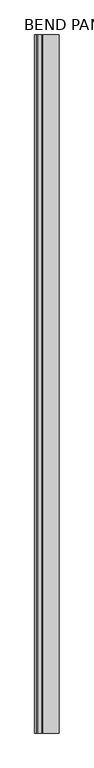
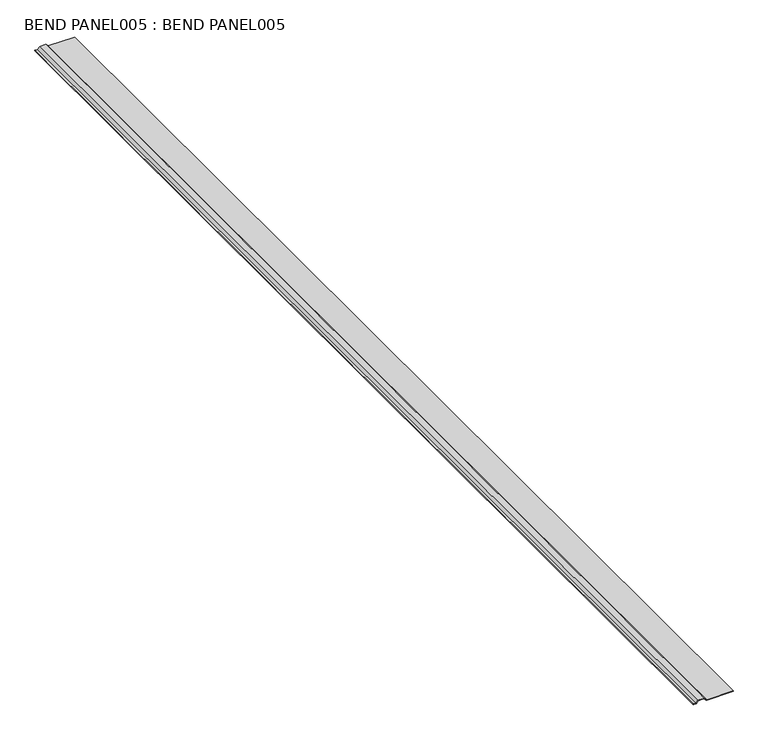
"""IFC4 building model written with IfcOpenShell, lengths in millimetres: proxy geometry, BEND PANEL005 : BEND PANEL005."""

import ifcopenshell
import ifcopenshell.guid

model = None  # the IFC model being written
_history = None  # IfcOwnerHistory: only IFC2X3 demands one
_inside = {}  # id of a spatial element -> (the spatial element, [elements in it])
_under = {}  # id of a project, library or spatial element -> (it, [spatial elements below it])
_declared = {}  # id of a project -> (the project, [libraries it declares])
_typed = {}  # id of a type object -> (the type object, [elements of that type])
_made_of = {}  # id of a material, layer set ... -> (it, [elements and type objects made of it])


def new_model(schema):
    """Start an empty IFC model of exactly this schema.

    Asked for "IFC4X3", IfcOpenShell would pick the latest addendum, in which some entities
    have other attributes; the version numbers below select the first issue.
    IFC2X3 requires an IfcOwnerHistory on every rooted entity: one is made here for all.
    """
    global model, _history
    if schema == "IFC4X3":
        model = ifcopenshell.file(schema_version=(4, 3, 0, 0))
    else:
        model = ifcopenshell.file(schema=schema)
    _inside.clear()
    _under.clear()
    _declared.clear()
    _typed.clear()
    _made_of.clear()
    _history = None
    if model.schema == "IFC2X3":
        org = make("IfcOrganization", Name="unknown")
        user = make(
            "IfcPersonAndOrganization",
            ThePerson=make("IfcPerson", FamilyName="unknown"),
            TheOrganization=org,
        )
        app = make(
            "IfcApplication",
            ApplicationDeveloper=org,
            Version="unknown",
            ApplicationFullName="unknown",
            ApplicationIdentifier="unknown",
        )
        _history = make(
            "IfcOwnerHistory",
            OwningUser=user,
            OwningApplication=app,
            ChangeAction="ADDED",
            CreationDate=0,
        )
    return model


def make(cls, **values):
    """One entity of the class cls with the attributes given. An attribute that is None is left unset."""
    return model.create_entity(
        cls, **{name: value for name, value in values.items() if value is not None}
    )


def rooted(cls, **values):
    """An entity with a GlobalId (a new one), such as an element, a storey or a relation."""
    return make(cls, GlobalId=ifcopenshell.guid.new(), OwnerHistory=_history, **values)


def si_unit(unit_type, name, prefix=None):
    """IfcSIUnit, for example si_unit("LENGTHUNIT", "METRE", prefix="MILLI")."""
    return make("IfcSIUnit", UnitType=unit_type, Prefix=prefix, Name=name)


def assignment(units):
    """IfcUnitAssignment: the units of a project."""
    return None if units is None else make("IfcUnitAssignment", Units=units)


def point(xyz):
    """IfcCartesianPoint."""
    return None if xyz is None else make("IfcCartesianPoint", Coordinates=xyz)


def direction(xyz):
    """IfcDirection."""
    return None if xyz is None else make("IfcDirection", DirectionRatios=xyz)


def frame(location, z_axis=None, x_axis=None):
    """IfcAxis2Placement3D, a coordinate frame: its origin and axes. An axis left out is left unset."""
    return make(
        "IfcAxis2Placement3D",
        Location=point(location),
        Axis=direction(z_axis),
        RefDirection=direction(x_axis),
    )


def frame_2d(location, x_axis=None):
    """IfcAxis2Placement2D, a coordinate frame in the plane: its origin and x axis."""
    return make(
        "IfcAxis2Placement2D", Location=point(location), RefDirection=direction(x_axis)
    )


def origin():
    """The frame at (0, 0, 0) with its axes left unset."""
    return frame((0.0, 0.0, 0.0))


def place(relative_to, where):
    """IfcLocalPlacement: puts the frame where relative to a parent placement (None: the world)."""
    return make(
        "IfcLocalPlacement", PlacementRelTo=relative_to, RelativePlacement=where
    )


def context(
    kind, dimensions, precision=None, world=None, true_north=None, identifier=None
):
    """IfcGeometricRepresentationContext, for example the 3D "Model" context."""
    return make(
        "IfcGeometricRepresentationContext",
        ContextIdentifier=identifier,
        ContextType=kind,
        CoordinateSpaceDimension=dimensions,
        Precision=precision,
        WorldCoordinateSystem=world,
        TrueNorth=true_north,
    )


def project(units=None, contexts=None):
    """IfcProject with its units and contexts."""
    return rooted(
        "IfcProject",
        Name="project",
        RepresentationContexts=contexts,
        UnitsInContext=assignment(units),
    )


def spatial(cls, under=None, at=None, **own):
    """A site, building, storey or space (cls), placed at a placement, below another one or the project."""
    s = rooted(cls, ObjectPlacement=at, **own)
    if under is not None:
        _under.setdefault(under.id(), (under, []))[1].append(s)
    return s


def polyline(points):
    """IfcPolyline through the points."""
    return make("IfcPolyline", Points=[point(p) for p in points])


def circle_curve(where, radius):
    """IfcCircle in the frame where."""
    return make("IfcCircle", Position=where, Radius=radius)


def trimmed(basis, trim1, trim2, sense, master):
    """IfcTrimmedCurve: the piece of a basis curve between two trims."""
    return make(
        "IfcTrimmedCurve",
        BasisCurve=basis,
        Trim1=trim1,
        Trim2=trim2,
        SenseAgreement=sense,
        MasterRepresentation=master,
    )


def segment(curve, same_sense, transition):
    """IfcCompositeCurveSegment."""
    return make(
        "IfcCompositeCurveSegment",
        Transition=transition,
        SameSense=same_sense,
        ParentCurve=curve,
    )


def composite_curve(segments, self_intersect=None):
    """IfcCompositeCurve: segments joined end to end."""
    return make("IfcCompositeCurve", Segments=segments, SelfIntersect=self_intersect)


def outline(outer, holes=None, kind="AREA"):
    """IfcArbitraryClosedProfileDef: a profile drawn as a closed curve; with holes, ...WithVoids."""
    if holes is None:
        return make("IfcArbitraryClosedProfileDef", ProfileType=kind, OuterCurve=outer)
    return make(
        "IfcArbitraryProfileDefWithVoids",
        ProfileType=kind,
        OuterCurve=outer,
        InnerCurves=holes,
    )


def extrude(swept, where, along, depth):
    """IfcExtrudedAreaSolid: the profile swept, set in the frame where, extruded along a direction by depth."""
    return make(
        "IfcExtrudedAreaSolid",
        SweptArea=swept,
        Position=where,
        ExtrudedDirection=direction(along),
        Depth=depth,
    )


def shape(context_of_items, identifier, shape_type, items):
    """IfcShapeRepresentation: the items that make up one representation, for example the "Body"."""
    return make(
        "IfcShapeRepresentation",
        ContextOfItems=context_of_items,
        RepresentationIdentifier=identifier,
        RepresentationType=shape_type,
        Items=items,
    )


def source(mapping_origin, context_of_items, identifier, shape_type, items):
    """IfcRepresentationMap: a shape defined once, which mapped items show again and again."""
    return make(
        "IfcRepresentationMap",
        MappingOrigin=mapping_origin,
        MappedRepresentation=shape(context_of_items, identifier, shape_type, items),
    )


def transform(
    local_origin,
    x_axis=None,
    y_axis=None,
    z_axis=None,
    scale=None,
    scale2=None,
    scale3=None,
    uniform=True,
):
    """IfcCartesianTransformationOperator3D, or its non-uniform kind. x_axis, y_axis, z_axis: its Axis1, 2, 3."""
    if uniform:
        return make(
            "IfcCartesianTransformationOperator3D",
            Axis1=direction(x_axis),
            Axis2=direction(y_axis),
            LocalOrigin=point(local_origin),
            Scale=scale,
            Axis3=direction(z_axis),
        )
    return make(
        "IfcCartesianTransformationOperator3DnonUniform",
        Axis1=direction(x_axis),
        Axis2=direction(y_axis),
        LocalOrigin=point(local_origin),
        Scale=scale,
        Axis3=direction(z_axis),
        Scale2=scale2,
        Scale3=scale3,
    )


def mapped(mapping_source, mapping_target):
    """IfcMappedItem: shows the shape of a source again, moved by a transform."""
    return make(
        "IfcMappedItem", MappingSource=mapping_source, MappingTarget=mapping_target
    )


def made_of(thing, what):
    """Note that an element or type object is made of a material, layer set ...; save() writes the relation."""
    if what is not None:
        _made_of.setdefault(what.id(), (what, []))[1].append(thing)
    return thing


def element(
    cls,
    number,
    at=None,
    inside=None,
    cuts=None,
    type_object=None,
    material=None,
    context=None,
    identifier="Body",
    shape_type=None,
    held_by="IfcProductDefinitionShape",
    body=None,
    shapes=None,
    **own,
):
    """One element of the class cls, such as IfcWall. Its Tag is "e" and its number.

    at: its placement. inside: the storey or other place that contains it. cuts: it is an
    opening in that element (IfcRelVoidsElement). A single representation is given by context,
    identifier, shape_type and body (its items); several are given by shapes. held_by: the class
    of the entity that holds the representations. save() writes the other relations.
    """
    e = rooted(cls, Tag="e%d" % number, ObjectPlacement=at, **own)
    if body is not None:
        shapes = [shape(context, identifier, shape_type, body)]
    if shapes is not None:
        e.Representation = make(held_by, Representations=shapes)
    if inside is not None:
        _inside.setdefault(inside.id(), (inside, []))[1].append(e)
    if cuts is not None:
        rooted(
            "IfcRelVoidsElement", RelatingBuildingElement=cuts, RelatedOpeningElement=e
        )
    if type_object is not None:
        _typed.setdefault(type_object.id(), (type_object, []))[1].append(e)
    return made_of(e, material)


def aggregate(whole, parts):
    """IfcRelAggregates: a whole, such as a stair, and the parts it consists of."""
    return rooted("IfcRelAggregates", RelatingObject=whole, RelatedObjects=parts)


def save(model, path):
    """Write the relations noted so far, then the file.

    IfcRelAggregates (storeys below a building ...), IfcRelContainedInSpatialStructure (elements
    in a storey), IfcRelDefinesByType, IfcRelAssociatesMaterial and IfcRelDeclares: one each for
    every whole, place, type object, material and project.
    """
    for whole, parts in _under.values():
        aggregate(whole, parts)
    for where, things in _inside.values():
        rooted(
            "IfcRelContainedInSpatialStructure",
            RelatedElements=things,
            RelatingStructure=where,
        )
    for kind, things in _typed.values():
        rooted("IfcRelDefinesByType", RelatedObjects=things, RelatingType=kind)
    for what, things in _made_of.values():
        rooted("IfcRelAssociatesMaterial", RelatedObjects=things, RelatingMaterial=what)
    for by, libraries in _declared.values():
        rooted("IfcRelDeclares", RelatingContext=by, RelatedDefinitions=libraries)
    model.write(path)


def bend_panel005_bend_panel005_8c87a596(model_context):
    return source(origin(), model_context, "Body", "SweptSolid", [
        extrude(outline(composite_curve([segment(polyline([(42575.4212949, 5895.2230694), (42576.6119199, 5895.2230694), (42576.6119199, 5848.7155886), (42580.7948046, 5844.5327039), (42580.7948046, 5833.5642507), (42576.6119199, 5829.381366), (42576.6119199, 5825.5083246), (42575.4212949, 5825.5083246), (42575.4212949, 5829.381366)]), True, "CONTINUOUS"), segment(trimmed(circle_curve(frame_2d((42576.6119199, 5829.381366)), 1.190625), [point((42575.4212949, 5829.381366))], [point((42575.7700209, 5830.223265))], False, "CARTESIAN"), True, "CONTINUOUS"), segment(polyline([(42575.7700209, 5830.223265), (42579.6041796, 5834.0574237), (42579.6041796, 5844.0395308), (42575.7700209, 5847.8736895)]), True, "CONTINUOUS"), segment(trimmed(circle_curve(frame_2d((42576.6119199, 5848.7155885)), 1.190625), [point((42575.7700209, 5847.8736895))], [point((42575.4212949, 5848.7155885))], False, "CARTESIAN"), True, "CONTINUOUS"), segment(polyline([(42575.4212949, 5848.7155885), (42575.4212949, 5895.2230694)]), True, "CONTINUOUS")], self_intersect=False)), frame((0.0, -1052.8906574, 0.0), z_axis=(0.0, 1.0, 0.0), x_axis=(0.0, 0.0, 1.0)), (0.0, 0.0, 1.0), 1999.85),
    ])


if __name__ == "__main__":
    model = new_model("IFC4")
    model_context = context("Model", 3, world=origin())
    ifc_project = project(units=[si_unit("LENGTHUNIT", "METRE", prefix="MILLI")], contexts=[model_context])
    site = spatial("IfcSite", under=ifc_project)
    building = spatial("IfcBuilding", under=site)
    placement = place(None, origin())
    bend_panel005_bend_panel005_shape = bend_panel005_bend_panel005_8c87a596(model_context)
    element("IfcBuildingElementProxy", 1, Name="BEND PANEL005 : BEND PANEL005", ObjectType="BEND PANEL005 : BEND PANEL005", at=placement, inside=building, context=model_context, shape_type="MappedRepresentation", body=[
        mapped(bend_panel005_bend_panel005_shape, transform((0.0, 0.0, 0.0), x_axis=(1.0, 0.0, 0.0), y_axis=(0.0, 1.0, 0.0), z_axis=(0.0, 0.0, 1.0))),
    ])
    save(model, "model.ifc")

# Revit data of these elements
# Type "BEND PANEL005 : BEND PANEL005"
#   NameOverride = "BEND PANEL005"
# Element 1 (IfcBuildingElementProxy, "BEND PANEL005 : BEND PANEL005")
#   Materials on its faces: "METAL PROFILE"
# Materials
#   "METAL PROFILE": class "Unassigned", colour RGB 128 128 128, transparency 0
